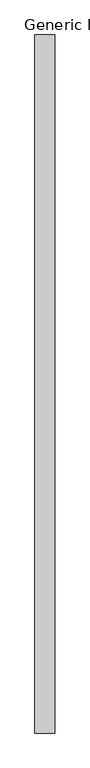
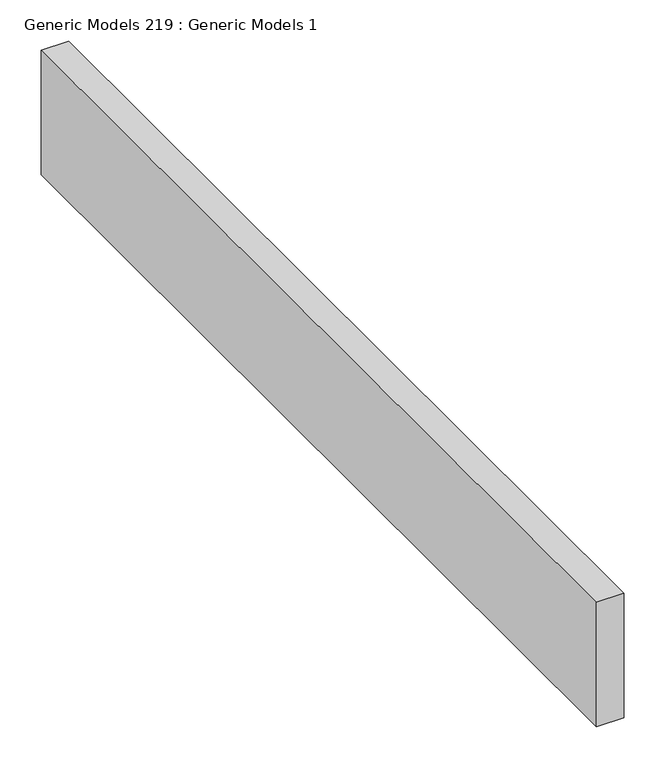
"""IFC4 building model written with IfcOpenShell, lengths in millimetres: proxy geometry, Generic Models 219 : Generic Models 1."""

from ifc_helpers import new_model, si_unit, frame, origin, place, context, project, spatial, polyline, outline, extrude, source, transform, mapped, element, save


def generic_models_219_generic_models_1_236455dc(model_context):
    return source(origin(), model_context, "Body", "SweptSolid", [
        extrude(outline(polyline([(-13578.5613975, -30595.7485041), (-13616.6613975, -30595.7485041), (-13616.6613975, -29249.5485041), (-13578.5613975, -29249.5485041), (-13578.5613975, -30595.7485041)])), frame((0.0, 0.0, 126625.096), z_axis=(0.0, 0.0, 1.0), x_axis=(1.0, 0.0, 0.0)), (0.0, 0.0, 1.0), 184.15),
    ])


if __name__ == "__main__":
    model = new_model("IFC4")
    model_context = context("Model", 3, world=origin())
    ifc_project = project(units=[si_unit("LENGTHUNIT", "METRE", prefix="MILLI")], contexts=[model_context])
    site = spatial("IfcSite", under=ifc_project)
    building = spatial("IfcBuilding", under=site)
    placement = place(None, origin())
    generic_models_219_generic_models_1_shape = generic_models_219_generic_models_1_236455dc(model_context)
    element("IfcBuildingElementProxy", 1, Name="Generic Models 219 : Generic Models 1", ObjectType="Generic Models 219 : Generic Models 1", at=placement, inside=building, context=model_context, shape_type="MappedRepresentation", body=[
        mapped(generic_models_219_generic_models_1_shape, transform((0.0, 0.0, 0.0), x_axis=(1.0, 0.0, 0.0), y_axis=(0.0, 1.0, 0.0), z_axis=(0.0, 0.0, 1.0))),
    ])
    save(model, "model.ifc")

# Revit data of these elements
# Element 1 (IfcBuildingElementProxy, "Generic Models 219 : Generic Models 1")
#   Materials on its faces: "_STRUCTURAL MEMBER (SEE STRUCT. DWGS)"
# Materials
#   "_STRUCTURAL MEMBER (SEE STRUCT. DWGS)": class "Generic", colour RGB 209 182 141, transparency 0, Cost = 0
